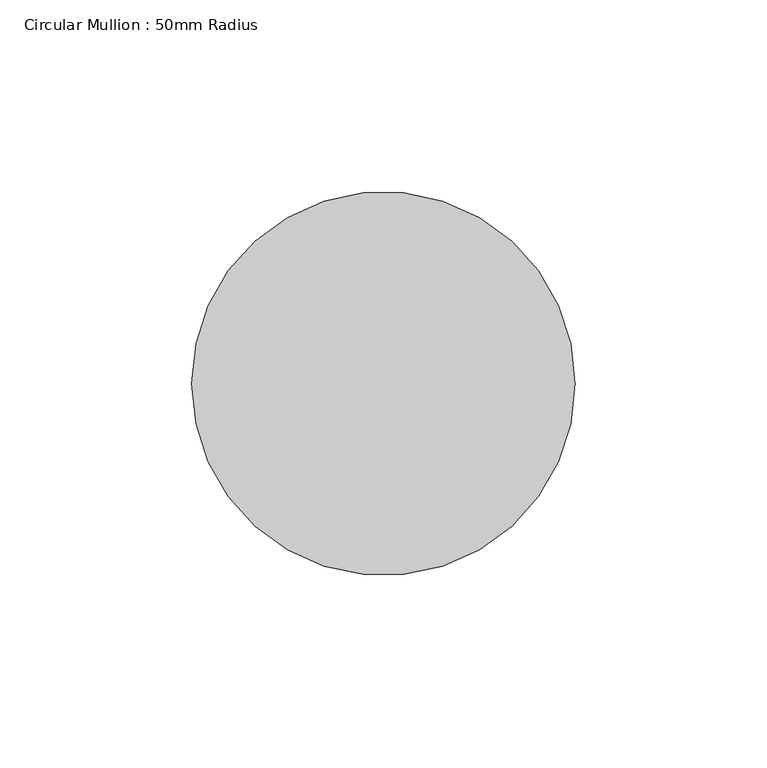
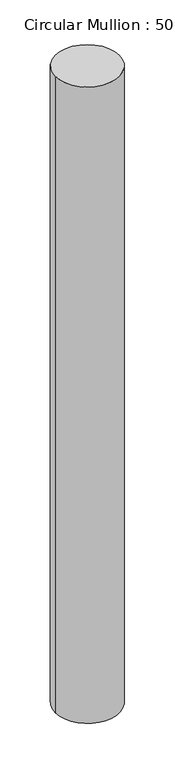
"""IFC4 building model written with IfcOpenShell, lengths in millimetres: member geometry, Circular Mullion : 50mm Radius."""

import ifcopenshell
import ifcopenshell.guid

model = None  # the IFC model being written
_history = None  # IfcOwnerHistory: only IFC2X3 demands one
_inside = {}  # id of a spatial element -> (the spatial element, [elements in it])
_under = {}  # id of a project, library or spatial element -> (it, [spatial elements below it])
_declared = {}  # id of a project -> (the project, [libraries it declares])
_typed = {}  # id of a type object -> (the type object, [elements of that type])
_made_of = {}  # id of a material, layer set ... -> (it, [elements and type objects made of it])


def new_model(schema):
    """Start an empty IFC model of exactly this schema.

    Asked for "IFC4X3", IfcOpenShell would pick the latest addendum, in which some entities
    have other attributes; the version numbers below select the first issue.
    IFC2X3 requires an IfcOwnerHistory on every rooted entity: one is made here for all.
    """
    global model, _history
    if schema == "IFC4X3":
        model = ifcopenshell.file(schema_version=(4, 3, 0, 0))
    else:
        model = ifcopenshell.file(schema=schema)
    _inside.clear()
    _under.clear()
    _declared.clear()
    _typed.clear()
    _made_of.clear()
    _history = None
    if model.schema == "IFC2X3":
        org = make("IfcOrganization", Name="unknown")
        user = make(
            "IfcPersonAndOrganization",
            ThePerson=make("IfcPerson", FamilyName="unknown"),
            TheOrganization=org,
        )
        app = make(
            "IfcApplication",
            ApplicationDeveloper=org,
            Version="unknown",
            ApplicationFullName="unknown",
            ApplicationIdentifier="unknown",
        )
        _history = make(
            "IfcOwnerHistory",
            OwningUser=user,
            OwningApplication=app,
            ChangeAction="ADDED",
            CreationDate=0,
        )
    return model


def make(cls, **values):
    """One entity of the class cls with the attributes given. An attribute that is None is left unset."""
    return model.create_entity(
        cls, **{name: value for name, value in values.items() if value is not None}
    )


def rooted(cls, **values):
    """An entity with a GlobalId (a new one), such as an element, a storey or a relation."""
    return make(cls, GlobalId=ifcopenshell.guid.new(), OwnerHistory=_history, **values)


def si_unit(unit_type, name, prefix=None):
    """IfcSIUnit, for example si_unit("LENGTHUNIT", "METRE", prefix="MILLI")."""
    return make("IfcSIUnit", UnitType=unit_type, Prefix=prefix, Name=name)


def assignment(units):
    """IfcUnitAssignment: the units of a project."""
    return None if units is None else make("IfcUnitAssignment", Units=units)


def point(xyz):
    """IfcCartesianPoint."""
    return None if xyz is None else make("IfcCartesianPoint", Coordinates=xyz)


def direction(xyz):
    """IfcDirection."""
    return None if xyz is None else make("IfcDirection", DirectionRatios=xyz)


def frame(location, z_axis=None, x_axis=None):
    """IfcAxis2Placement3D, a coordinate frame: its origin and axes. An axis left out is left unset."""
    return make(
        "IfcAxis2Placement3D",
        Location=point(location),
        Axis=direction(z_axis),
        RefDirection=direction(x_axis),
    )


def frame_2d(location, x_axis=None):
    """IfcAxis2Placement2D, a coordinate frame in the plane: its origin and x axis."""
    return make(
        "IfcAxis2Placement2D", Location=point(location), RefDirection=direction(x_axis)
    )


def origin():
    """The frame at (0, 0, 0) with its axes left unset."""
    return frame((0.0, 0.0, 0.0))


def origin_2d():
    """The frame at (0, 0) in the plane with its x axis left unset."""
    return frame_2d((0.0, 0.0))


def place(relative_to, where):
    """IfcLocalPlacement: puts the frame where relative to a parent placement (None: the world)."""
    return make(
        "IfcLocalPlacement", PlacementRelTo=relative_to, RelativePlacement=where
    )


def context(
    kind, dimensions, precision=None, world=None, true_north=None, identifier=None
):
    """IfcGeometricRepresentationContext, for example the 3D "Model" context."""
    return make(
        "IfcGeometricRepresentationContext",
        ContextIdentifier=identifier,
        ContextType=kind,
        CoordinateSpaceDimension=dimensions,
        Precision=precision,
        WorldCoordinateSystem=world,
        TrueNorth=true_north,
    )


def project(units=None, contexts=None):
    """IfcProject with its units and contexts."""
    return rooted(
        "IfcProject",
        Name="project",
        RepresentationContexts=contexts,
        UnitsInContext=assignment(units),
    )


def spatial(cls, under=None, at=None, **own):
    """A site, building, storey or space (cls), placed at a placement, below another one or the project."""
    s = rooted(cls, ObjectPlacement=at, **own)
    if under is not None:
        _under.setdefault(under.id(), (under, []))[1].append(s)
    return s


def circle_curve(where, radius):
    """IfcCircle in the frame where."""
    return make("IfcCircle", Position=where, Radius=radius)


def trimmed(basis, trim1, trim2, sense, master):
    """IfcTrimmedCurve: the piece of a basis curve between two trims."""
    return make(
        "IfcTrimmedCurve",
        BasisCurve=basis,
        Trim1=trim1,
        Trim2=trim2,
        SenseAgreement=sense,
        MasterRepresentation=master,
    )


def segment(curve, same_sense, transition):
    """IfcCompositeCurveSegment."""
    return make(
        "IfcCompositeCurveSegment",
        Transition=transition,
        SameSense=same_sense,
        ParentCurve=curve,
    )


def composite_curve(segments, self_intersect=None):
    """IfcCompositeCurve: segments joined end to end."""
    return make("IfcCompositeCurve", Segments=segments, SelfIntersect=self_intersect)


def outline(outer, holes=None, kind="AREA"):
    """IfcArbitraryClosedProfileDef: a profile drawn as a closed curve; with holes, ...WithVoids."""
    if holes is None:
        return make("IfcArbitraryClosedProfileDef", ProfileType=kind, OuterCurve=outer)
    return make(
        "IfcArbitraryProfileDefWithVoids",
        ProfileType=kind,
        OuterCurve=outer,
        InnerCurves=holes,
    )


def extrude(swept, where, along, depth):
    """IfcExtrudedAreaSolid: the profile swept, set in the frame where, extruded along a direction by depth."""
    return make(
        "IfcExtrudedAreaSolid",
        SweptArea=swept,
        Position=where,
        ExtrudedDirection=direction(along),
        Depth=depth,
    )


def shape(context_of_items, identifier, shape_type, items):
    """IfcShapeRepresentation: the items that make up one representation, for example the "Body"."""
    return make(
        "IfcShapeRepresentation",
        ContextOfItems=context_of_items,
        RepresentationIdentifier=identifier,
        RepresentationType=shape_type,
        Items=items,
    )


def source(mapping_origin, context_of_items, identifier, shape_type, items):
    """IfcRepresentationMap: a shape defined once, which mapped items show again and again."""
    return make(
        "IfcRepresentationMap",
        MappingOrigin=mapping_origin,
        MappedRepresentation=shape(context_of_items, identifier, shape_type, items),
    )


def transform(
    local_origin,
    x_axis=None,
    y_axis=None,
    z_axis=None,
    scale=None,
    scale2=None,
    scale3=None,
    uniform=True,
):
    """IfcCartesianTransformationOperator3D, or its non-uniform kind. x_axis, y_axis, z_axis: its Axis1, 2, 3."""
    if uniform:
        return make(
            "IfcCartesianTransformationOperator3D",
            Axis1=direction(x_axis),
            Axis2=direction(y_axis),
            LocalOrigin=point(local_origin),
            Scale=scale,
            Axis3=direction(z_axis),
        )
    return make(
        "IfcCartesianTransformationOperator3DnonUniform",
        Axis1=direction(x_axis),
        Axis2=direction(y_axis),
        LocalOrigin=point(local_origin),
        Scale=scale,
        Axis3=direction(z_axis),
        Scale2=scale2,
        Scale3=scale3,
    )


def mapped(mapping_source, mapping_target):
    """IfcMappedItem: shows the shape of a source again, moved by a transform."""
    return make(
        "IfcMappedItem", MappingSource=mapping_source, MappingTarget=mapping_target
    )


def made_of(thing, what):
    """Note that an element or type object is made of a material, layer set ...; save() writes the relation."""
    if what is not None:
        _made_of.setdefault(what.id(), (what, []))[1].append(thing)
    return thing


def element(
    cls,
    number,
    at=None,
    inside=None,
    cuts=None,
    type_object=None,
    material=None,
    context=None,
    identifier="Body",
    shape_type=None,
    held_by="IfcProductDefinitionShape",
    body=None,
    shapes=None,
    **own,
):
    """One element of the class cls, such as IfcWall. Its Tag is "e" and its number.

    at: its placement. inside: the storey or other place that contains it. cuts: it is an
    opening in that element (IfcRelVoidsElement). A single representation is given by context,
    identifier, shape_type and body (its items); several are given by shapes. held_by: the class
    of the entity that holds the representations. save() writes the other relations.
    """
    e = rooted(cls, Tag="e%d" % number, ObjectPlacement=at, **own)
    if body is not None:
        shapes = [shape(context, identifier, shape_type, body)]
    if shapes is not None:
        e.Representation = make(held_by, Representations=shapes)
    if inside is not None:
        _inside.setdefault(inside.id(), (inside, []))[1].append(e)
    if cuts is not None:
        rooted(
            "IfcRelVoidsElement", RelatingBuildingElement=cuts, RelatedOpeningElement=e
        )
    if type_object is not None:
        _typed.setdefault(type_object.id(), (type_object, []))[1].append(e)
    return made_of(e, material)


def aggregate(whole, parts):
    """IfcRelAggregates: a whole, such as a stair, and the parts it consists of."""
    return rooted("IfcRelAggregates", RelatingObject=whole, RelatedObjects=parts)


def save(model, path):
    """Write the relations noted so far, then the file.

    IfcRelAggregates (storeys below a building ...), IfcRelContainedInSpatialStructure (elements
    in a storey), IfcRelDefinesByType, IfcRelAssociatesMaterial and IfcRelDeclares: one each for
    every whole, place, type object, material and project.
    """
    for whole, parts in _under.values():
        aggregate(whole, parts)
    for where, things in _inside.values():
        rooted(
            "IfcRelContainedInSpatialStructure",
            RelatedElements=things,
            RelatingStructure=where,
        )
    for kind, things in _typed.values():
        rooted("IfcRelDefinesByType", RelatedObjects=things, RelatingType=kind)
    for what, things in _made_of.values():
        rooted("IfcRelAssociatesMaterial", RelatedObjects=things, RelatingMaterial=what)
    for by, libraries in _declared.values():
        rooted("IfcRelDeclares", RelatingContext=by, RelatedDefinitions=libraries)
    model.write(path)


def circular_mullion_50mm_radius_3869dc77(model_context):
    return source(origin(), model_context, "Body", "SweptSolid", [
        extrude(outline(composite_curve([segment(trimmed(circle_curve(origin_2d(), 50.0), [point((50.0, 0.0))], [point((-50.0, 0.0))], False, "CARTESIAN"), True, "CONTINUOUS"), segment(trimmed(circle_curve(origin_2d(), 50.0), [point((-50.0, 0.0))], [point((50.0, 0.0))], False, "CARTESIAN"), True, "CONTINUOUS")], self_intersect=False)), frame((0.0, 0.0, -1052.692192), z_axis=(0.0, 0.0, 1.0), x_axis=(1.0, 0.0, 0.0)), (0.0, 0.0, 1.0), 1052.692192),
    ])


if __name__ == "__main__":
    model = new_model("IFC4")
    model_context = context("Model", 3, world=origin())
    ifc_project = project(units=[si_unit("LENGTHUNIT", "METRE", prefix="MILLI")], contexts=[model_context])
    site = spatial("IfcSite", under=ifc_project)
    building = spatial("IfcBuilding", under=site)
    placement = place(None, origin())
    circular_mullion_50mm_radius_shape = circular_mullion_50mm_radius_3869dc77(model_context)
    element("IfcMember", 1, ObjectType="Circular Mullion : 50mm Radius", at=placement, inside=building, context=model_context, shape_type="MappedRepresentation", body=[
        mapped(circular_mullion_50mm_radius_shape, transform((0.0, 0.0, 0.0), x_axis=(1.0, 0.0, 0.0), y_axis=(0.0, 1.0, 0.0), z_axis=(0.0, 0.0, 1.0))),
    ])
    save(model, "model.ifc")

# Revit data of these elements
# Type "Circular Mullion : 50mm Radius"
#   built-in parameter 1007350 = 0.164042 (stored number, unit not read)
# Element 1 (IfcMember, "Circular Mullion : 50mm Radius")
#   Materials on its faces: "Aluminium"
# Materials
#   "Aluminium": class "Metal", colour RGB 247 247 247, transparency 0, Description = "Aluminium 6061", Cost = 0
